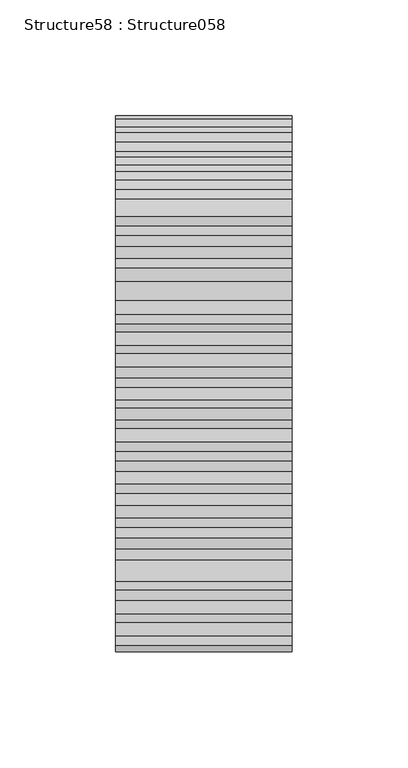
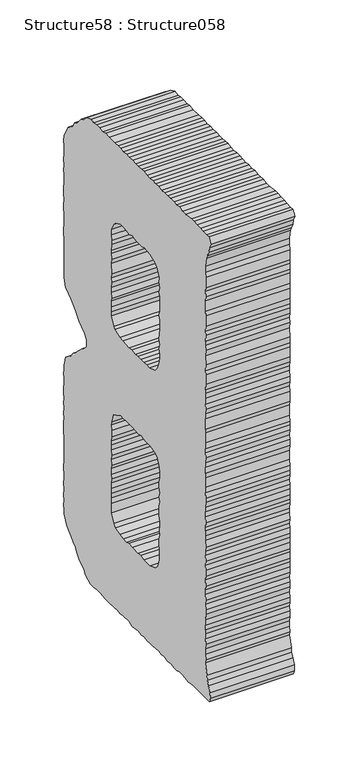
"""IFC4 building model written with IfcOpenShell, lengths in millimetres: proxy geometry, Structure58 : Structure058."""

from ifc_helpers import new_model, si_unit, frame, origin, place, context, project, spatial, polyline, outline, extrude, source, transform, mapped, element, save


def structure58_structure058_0e822dfb(model_context):
    return source(origin(), model_context, "Body", "SweptSolid", [
        extrude(outline(polyline([(258305.3557189, 3581.5276686), (258301.2543498, 3578.0103756), (258298.3355743, 3574.5107332), (258294.2117407, 3572.1423369), (258292.473954, 3568.6426945), (258288.3501205, 3563.9412034), (258284.8520827, 3561.025637), (258280.7282491, 3558.684519), (258278.4112002, 3554.5831499), (258270.7893289, 3550.4833855), (258264.9277087, 3551.0658569), (258260.2486819, 3551.6675836), (258255.5680506, 3551.6675836), (258252.0250839, 3551.0658569), (258247.3444526, 3550.4833855), (258242.0620946, 3551.0658569), (258232.7024366, 3551.0658569), (258227.9993408, 3551.6675836), (258224.501303, 3550.4833855), (258219.218945, 3551.6675836), (258210.4385492, 3551.6675836), (258205.1561912, 3550.4833855), (258201.0564267, 3550.4833855), (258195.7965332, 3551.6675836), (258190.5141752, 3550.4833855), (258186.9936729, 3551.0658569), (258181.1545171, 3550.4833855), (258177.6324103, 3551.0658569), (258172.9533836, 3551.0658569), (258167.6485611, 3551.6675836), (258164.1505233, 3551.6675836), (258159.4474275, 3550.4833855), (258154.7667962, 3551.6675836), (258149.5085073, 3550.4833855), (258144.2261493, 3551.0658569), (258139.545518, 3550.4833855), (258134.8664913, 3550.4833855), (258130.7426577, 3551.6675836), (258126.6428932, 3551.6675836), (258121.3605352, 3551.0658569), (258117.2816306, 3550.4833855), (258112.0008772, 3551.0658569), (258107.8995081, 3551.6675836), (258083.8753696, 3551.6675836), (258082.1151185, 3555.7416744), (258082.7168452, 3561.025637), (258085.033894, 3566.3095996), (258086.7941452, 3570.4109687), (258087.3958719, 3574.5107332), (258090.3387165, 3585.0706354), (258089.1577276, 3588.5702778), (258090.3387165, 3593.2541183), (258090.3387165, 3598.5284533), (258089.1577276, 3603.2122938), (258089.7369898, 3608.4705827), (258090.3387165, 3612.5976255), (258089.7369898, 3616.69739), (258089.7369898, 3621.3732075), (258090.3387165, 3626.0554434), (258089.1577276, 3631.915459), (258089.1577276, 3636.6153456), (258090.3387165, 3640.7167147), (258089.1577276, 3645.4262289), (258089.7369898, 3650.6845178), (258089.7369898, 3655.3587307), (258089.1577276, 3658.8840468), (258089.7369898, 3664.7440624), (258089.1577276, 3668.2437048), (258089.1577276, 3674.1277895), (258089.7369898, 3678.81163), (258089.1577276, 3682.8857208), (258089.7369898, 3688.1873341), (258090.3387165, 3691.6869765), (258089.1577276, 3696.3884676), (258090.3387165, 3702.229228), (258090.3387165, 3706.3289925), (258089.7369898, 3711.6145597), (258089.7369898, 3715.1302482), (258089.1577276, 3719.8140887), (258089.7369898, 3725.0996559), (258089.7369898, 3729.7738688), (258090.3387165, 3733.8736333), (258089.1577276, 3739.1592005), (258089.1577276, 3743.2332913), (258089.7369898, 3747.9428055), (258090.3387165, 3753.2171405), (258090.3387165, 3762.0023501), (258089.7369898, 3766.684586), (258089.7369898, 3772.5606477), (258090.3387165, 3776.6427615), (258089.1577276, 3781.9299333), (258089.7369898, 3786.6298199), (258089.7369898, 3790.1294623), (258090.3387165, 3795.4037973), (258090.3387165, 3805.3459267), (258089.7369898, 3808.8888934), (258089.7369898, 3818.8310229), (258090.3387165, 3823.5341187), (258089.1577276, 3828.2163546), (258089.7369898, 3832.8921721), (258090.3387165, 3838.1761347), (258090.3387165, 3842.8583706), (258089.7369898, 3846.9757858), (258089.1577276, 3852.2340747), (258089.1577276, 3861.6178018), (258089.7369898, 3865.1190488), (258089.1577276, 3870.9790644), (258090.3387165, 3879.1769888), (258089.1577276, 3885.0626781), (258090.3387165, 3889.1463965), (258089.7369898, 3893.246161), (258089.1577276, 3899.1061766), (258089.7369898, 3902.6314927), (258089.1577276, 3907.888177), (258089.1577276, 3917.8479571), (258089.7369898, 3921.9733953), (258089.7369898, 3931.9058971), (258089.1577276, 3936.0345445), (258089.7369898, 3941.2912288), (258089.1577276, 3944.8165449), (258089.1577276, 3954.7506513), (258090.3387165, 3958.8776941), (258090.3387165, 3964.7361051), (258088.5560009, 3973.5197101), (258086.7941452, 3977.0209571), (258084.4546318, 3981.7208437), (258083.8753696, 3986.4046842), (258081.5358562, 3991.0788971), (258084.4546318, 3996.390138), (258088.5560009, 3995.7803883), (258094.4160165, 3995.7803883), (258097.9381234, 3996.390138), (258103.7997436, 3996.390138), (258108.4787703, 3996.9645864), (258112.0008772, 3996.9645864), (258121.3605352, 3995.7803883), (258126.063631, 3995.7803883), (258130.7426577, 3996.9645864), (258135.4457535, 3996.390138), (258139.545518, 3996.390138), (258144.8054115, 3996.9645864), (258150.0877695, 3995.7803883), (258154.187534, 3996.390138), (258159.4474275, 3995.7803883), (258164.1505233, 3996.390138), (258168.2502878, 3996.390138), (258172.3516569, 3996.9645864), (258178.2132771, 3995.7803883), (258181.7113149, 3996.390138), (258186.9936729, 3996.9645864), (258190.5141752, 3996.9645864), (258195.7965332, 3996.390138), (258199.8962977, 3996.390138), (258204.576929, 3996.9645864), (258210.4385492, 3996.390138), (258213.936587, 3996.9645864), (258219.7982072, 3995.7803883), (258223.3203141, 3996.9645864), (258227.4200786, 3996.9645864), (258233.3041633, 3996.390138), (258241.4828324, 3996.390138), (258247.3444526, 3996.9645864), (258251.4442171, 3995.7803883), (258256.7041106, 3996.390138), (258261.4072064, 3996.390138), (258265.5069709, 3995.7803883), (258269.60834, 3996.9645864), (258277.2302113, 3993.4472933), (258281.3299758, 3989.3475288), (258285.4313449, 3987.0048063), (258288.9518472, 3982.8793681), (258291.8722273, 3979.3781211), (258295.3927296, 3977.6194746), (258297.7338476, 3972.9372387), (258301.8336121, 3969.994394), (258305.9349811, 3967.0788276), (258308.296959, 3962.9774586), (258311.7966014, 3955.9348494), (258312.9775903, 3950.0940891), (258311.7966014, 3945.9766739), (258311.7966014, 3940.718385), (258312.3758636, 3937.1930689), (258312.9775903, 3932.4899731), (258312.3758636, 3926.6492128), (258312.9775903, 3921.9733953), (258312.3758636, 3917.8479571), (258311.7966014, 3912.5896682), (258312.9775903, 3903.2059411), (258312.9775903, 3899.1061766), (258312.3758636, 3893.822214), (258312.9775903, 3889.7208449), (258312.9775903, 3885.6210804), (258311.7966014, 3880.3627915), (258311.7966014, 3875.686974), (258312.3758636, 3870.4030114), (258312.9775903, 3865.7015202), (258312.9775903, 3861.0192843), (258312.3758636, 3856.9179152), (258312.3758636, 3851.6612309), (258311.7966014, 3847.5598618), (258311.7966014, 3823.5341187), (258312.3758636, 3819.4150989), (258309.4554834, 3811.2043377), (258304.7764567, 3808.290376), (258301.2543498, 3805.3459267), (258297.7338476, 3802.448011), (258294.2117407, 3798.3305959), (258291.2929651, 3794.2292268), (258288.3501205, 3791.8865042), (258284.8520827, 3788.9452642), (258280.1489869, 3785.4456218), (258277.2302113, 3780.7441306), (258277.2302113, 3774.3032481), (258280.1489869, 3770.8036057), (258283.6710938, 3768.4432325), (258287.7708583, 3764.3611187), (258291.2929651, 3761.418274), (258294.7910029, 3757.3185096), (258298.3355743, 3754.9854146), (258301.8336121, 3750.3015741), (258305.3557189, 3747.9428055), (258309.4554834, 3744.4158848), (258311.7966014, 3735.6146291), (258311.7966014, 3730.9323932), (258312.9775903, 3727.4311462), (258312.3758636, 3722.7312597), (258312.3758636, 3718.0554422), (258312.9775903, 3713.3555556), (258312.9775903, 3708.087639), (258312.3758636, 3703.4134261), (258312.9775903, 3698.711935), (258311.7966014, 3694.6298211), (258312.9775903, 3689.3458585), (258312.3758636, 3684.6443673), (258312.9775903, 3681.1447249), (258312.9775903, 3670.5848228), (258311.7966014, 3666.5027089), (258311.7966014, 3644.2420307), (258312.9775903, 3638.3563415), (258311.7966014, 3628.998288), (258312.9775903, 3621.3732075), (258312.3758636, 3616.69739), (258312.9775903, 3610.838979), (258311.7966014, 3606.1551384), (258312.9775903, 3601.4536473), (258311.7966014, 3597.3538828), (258311.7966014, 3593.2541183), (258308.296959, 3585.0706354), (258305.3557189, 3581.5276686)]), holes=[polyline([(258237.3830679, 3831.732043), (258237.9847946, 3836.4174882), (258237.9847946, 3842.2758992), (258236.8022011, 3845.1914656), (258237.9847946, 3850.4754282), (258237.9847946, 3855.1769193), (258236.8022011, 3860.4432313), (258237.9847946, 3863.9332461), (258236.8022011, 3868.6443649), (258237.9847946, 3878.0024183), (258236.8022011, 3882.7039095), (258237.3830679, 3887.9621984), (258237.3830679, 3890.905043), (258236.8022011, 3896.763454), (258236.8022011, 3900.8648231), (258237.3830679, 3905.5470591), (258237.3830679, 3910.8310217), (258233.860961, 3917.8479571), (258231.5214477, 3920.2067257), (258223.9220408, 3923.7079727), (258219.7982072, 3923.7079727), (258215.1191805, 3923.1319197), (258209.859287, 3922.5494483), (258205.7354534, 3923.7079727), (258199.8962977, 3922.5494483), (258190.5141752, 3922.5494483), (258186.9936729, 3923.7079727), (258182.3130416, 3923.7079727), (258177.6324103, 3923.1319197), (258169.4088122, 3919.6066036), (258165.9107744, 3916.6653636), (258162.9695344, 3909.6468235), (258163.5712611, 3904.9645876), (258162.3886676, 3900.2887701), (258163.5712611, 3895.5888836), (258162.3886676, 3892.0876365), (258162.3886676, 3878.0024183), (258163.5712611, 3873.3185778), (258162.3886676, 3869.2444869), (258162.3886676, 3860.4432313), (258163.5712611, 3851.0595042), (258162.3886676, 3845.8012153), (258163.5712611, 3841.6741725), (258162.3886676, 3836.4174882), (258162.3886676, 3832.8921721), (258163.5712611, 3827.0321565), (258166.4900367, 3820.5896694), (258169.4088122, 3817.090027), (258177.6324103, 3814.7296538), (258181.7113149, 3814.7296538), (258186.9936729, 3814.148787), (258191.6726996, 3814.148787), (258195.7965332, 3814.7296538), (258199.8962977, 3814.148787), (258205.7354534, 3814.7296538), (258209.859287, 3814.148787), (258219.218945, 3815.3313805), (258224.501303, 3815.3313805), (258232.1231743, 3818.2309008), (258233.860961, 3820.015221), (258237.9847946, 3827.6162325), (258237.3830679, 3831.732043)]), polyline([(258230.9421854, 3736.7988273), (258223.3203141, 3740.9162424), (258219.7982072, 3740.3161203), (258215.1191805, 3740.3161203), (258209.859287, 3740.9162424), (258205.7354534, 3740.3161203), (258200.4771645, 3740.3161203), (258195.7965332, 3739.7416719), (258191.6726996, 3740.9162424), (258185.8351485, 3739.7416719), (258177.0306836, 3739.7416719), (258169.4088122, 3737.400554), (258166.4900367, 3735.0578314), (258162.9695344, 3728.0152223), (258162.3886676, 3723.3313817), (258162.3886676, 3718.0554422), (258163.5712611, 3713.3555556), (258163.5712611, 3709.2718371), (258162.3886676, 3703.4134261), (258163.5712611, 3699.3136616), (258162.3886676, 3695.2122926), (258163.5712611, 3690.512406), (258163.5712611, 3681.7271964), (258162.3886676, 3676.4432338), (258162.3886676, 3671.7690209), (258162.9695344, 3667.6853024), (258162.3886676, 3663.5598643), (258163.5712611, 3658.8840468), (258163.5712611, 3654.1841602), (258162.9695344, 3648.9258713), (258162.9695344, 3639.5405396), (258165.3315122, 3631.915459), (258168.82955, 3628.4158166), (258177.0306836, 3625.472972), (258186.4144107, 3625.472972), (258191.0934374, 3626.6571701), (258195.7965332, 3626.0554434), (258204.576929, 3626.0554434), (258209.859287, 3626.6571701), (258213.936587, 3625.472972), (258218.6396828, 3626.0554434), (258224.501303, 3626.6571701), (258231.5214477, 3628.4158166), (258233.860961, 3631.3410106), (258237.3830679, 3639.5405396), (258237.3830679, 3648.3161216), (258237.9847946, 3653.6000842), (258237.3830679, 3658.3015753), (258237.3830679, 3662.9854159), (258237.9847946, 3667.6853024), (258236.8022011, 3672.3691429), (258237.3830679, 3676.4432338), (258237.9847946, 3681.7271964), (258236.8022011, 3685.2444894), (258237.9847946, 3690.512406), (258236.8022011, 3694.6298211), (258237.9847946, 3699.3136616), (258237.3830679, 3704.5879966), (258237.9847946, 3708.087639), (258236.8022011, 3712.7971532), (258236.8022011, 3718.6571688), (258237.9847946, 3723.3313817), (258236.8022011, 3726.8566978), (258234.4402232, 3735.0578314), (258230.9421854, 3736.7988273)])]), frame((-38594.2176606, 0.0, 0.0), z_axis=(1.0, 0.0, 0.0), x_axis=(0.0, 1.0, 0.0)), (0.0, 0.0, 1.0), 76.2),
    ])


if __name__ == "__main__":
    model = new_model("IFC4")
    model_context = context("Model", 3, world=origin())
    ifc_project = project(units=[si_unit("LENGTHUNIT", "METRE", prefix="MILLI")], contexts=[model_context])
    site = spatial("IfcSite", under=ifc_project)
    building = spatial("IfcBuilding", under=site)
    placement = place(None, origin())
    structure58_structure058_shape = structure58_structure058_0e822dfb(model_context)
    element("IfcBuildingElementProxy", 1, Name="Structure58 : Structure058", ObjectType="Structure58 : Structure058", at=placement, inside=building, context=model_context, shape_type="MappedRepresentation", body=[
        mapped(structure58_structure058_shape, transform((0.0, 0.0, 0.0), x_axis=(1.0, 0.0, 0.0), y_axis=(0.0, 1.0, 0.0), z_axis=(0.0, 0.0, 1.0))),
    ])
    save(model, "model.ifc")

# Revit data of these elements
# Type "Structure58 : Structure058"
#   NameOverride = "Structure058"
# Element 1 (IfcBuildingElementProxy, "Structure58 : Structure058")
#   Materials on its faces: "BRUSHED ALUM. LETTERING"
# Materials
#   "BRUSHED ALUM. LETTERING": class "Unassigned", colour RGB 169 181 186, transparency 0, Cost = 0
